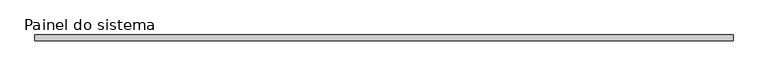
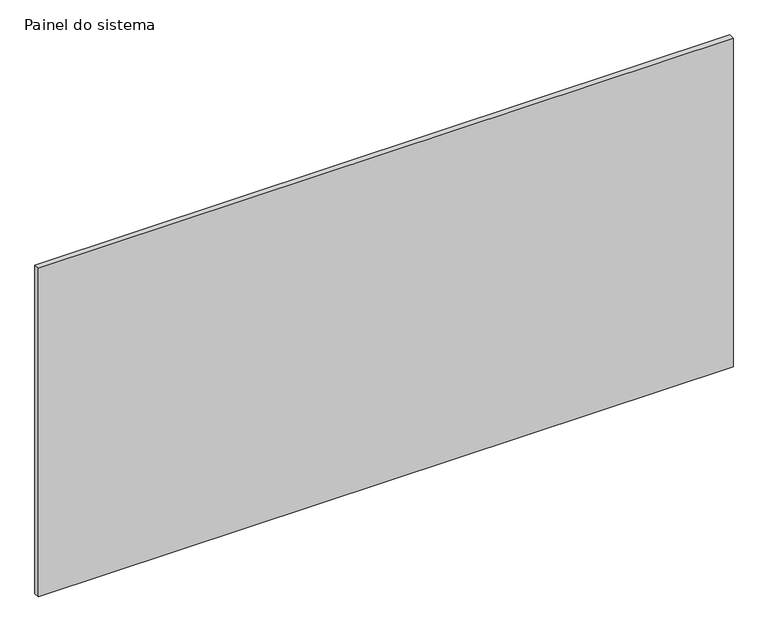
"""IFC4 building model written with IfcOpenShell, lengths in millimetres: plate geometry, Painel do sistema : Envidraçado."""

from ifc_helpers import new_model, si_unit, origin, origin_with_axes, place, context, project, spatial, polyline, outline, extrude, source, transform, mapped, element, save


def painel_do_sistema_1cdad03e(model_context):
    return source(origin(), model_context, "Body", "SweptSolid", [
        extrude(outline(polyline([(1500.0, 24.5), (-1500.0, 24.5), (-1500.0, 49.5), (1500.0, 49.5), (1500.0, 24.5)])), origin_with_axes(), (0.0, 0.0, 1.0), 1500.0),
    ])


if __name__ == "__main__":
    model = new_model("IFC4")
    model_context = context("Model", 3, world=origin())
    ifc_project = project(units=[si_unit("LENGTHUNIT", "METRE", prefix="MILLI")], contexts=[model_context])
    site = spatial("IfcSite", under=ifc_project)
    building = spatial("IfcBuilding", under=site)
    placement = place(None, origin())
    painel_do_sistema_shape = painel_do_sistema_1cdad03e(model_context)
    element("IfcPlate", 1, ObjectType="Painel do sistema : Envidraçado", at=placement, inside=building, context=model_context, shape_type="MappedRepresentation", body=[
        mapped(painel_do_sistema_shape, transform((0.0, 0.0, 0.0), x_axis=(1.0, 0.0, 0.0), y_axis=(0.0, 1.0, 0.0), z_axis=(0.0, 0.0, 1.0))),
    ])
    save(model, "model.ifc")

# Revit data of these elements
# Type "Painel do sistema : Envidraçado"
#   Construction Type Id = "GSP4R"
#   Analytic Construction = "Vidraça única Pilkington 1/8 pol"
#   Visual Light Transmittance = 0.9
#   Solar Heat Gain Coefficient = 0.86
#   Heat Transfer Coefficient (U) = 6.7069 W/(m²·K)
# Element 1 (IfcPlate, "Painel do sistema : Envidraçado")
#   Materials on its faces: "Vidro"
# Materials
#   "Vidro": class "Vidro", colour RGB 0 128 192, transparency 0.9, Description = "Vidro de sílica", Cost = 0
